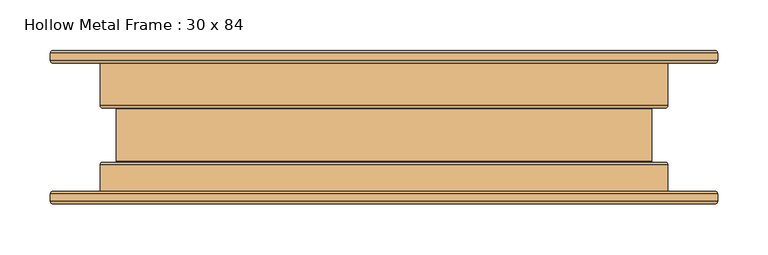
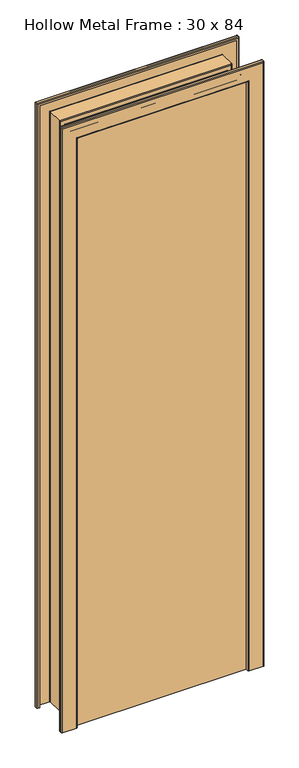
"""IFC4 building model written with IfcOpenShell, lengths in millimetres: door geometry, Hollow Metal Frame : 30 x 84."""

from ifc_helpers import new_model, si_unit, frame, origin, origin_with_axes, place, context, project, spatial, polyline, circle_curve, ellipse_curve, outline, extrude, source, transform, mapped, element, save
from ifc_brep_helpers import plane_surface, cylinder_surface, revolved_surface, advanced_brep


def hollow_metal_frame_30_x_84_32adf456(model_context):
    return source(origin(), model_context, "Body", "SolidModel", [
        advanced_brep(
        [(-327.62825, 63.5635, 0.0), (-330.2, 66.13525, 0.0), (-330.2, 73.66, 0.0), (-327.62825, 76.23175, 0.0), (-281.97175, 76.23175, 0.0), (-279.4, 73.66, 0.0), (-279.4, 21.68525, 0.0), (-278.384, 20.66925, 0.0), (-266.09675, 20.66925, 0.0), (-263.525, 18.0975, 0.0), (-263.525, -33.6931, 0.0), (-266.09675, -36.26485, 0.0), (-278.384, -36.26485, 0.0), (-279.4, -37.28085, 0.0), (-279.4, -73.5965, 0.0), (-281.97175, -76.16825, 0.0), (-327.62825, -76.16825, 0.0), (-330.2, -73.5965, 0.0), (-330.2, -66.07175, 0.0), (-327.62825, -63.5, 0.0), (-322.2625, -63.5, 0.0), (-322.2625, -65.05575, 0.0), (-327.62825, -65.05575, 0.0), (-328.64425, -66.07175, 0.0), (-328.64425, -73.5965, 0.0), (-327.62825, -74.6125, 0.0), (-281.97175, -74.6125, 0.0), (-280.95575, -73.5965, 0.0), (-280.95575, -37.28085, 0.0), (-278.384, -34.7091, 0.0), (-266.09675, -34.7091, 0.0), (-265.08075, -33.6931, 0.0), (-265.08075, 18.0975, 0.0), (-266.09675, 19.1135, 0.0), (-278.384, 19.1135, 0.0), (-280.95575, 21.68525, 0.0), (-280.95575, 73.66, 0.0), (-281.97175, 74.676, 0.0), (-327.62825, 74.676, 0.0), (-328.64425, 73.66, 0.0), (-328.64425, 66.13525, 0.0), (-327.62825, 65.11925, 0.0), (-322.2625, 65.11925, 0.0), (-322.2625, 63.5635, 0.0), (-327.62825, 63.5635, 2080.2282501), (-330.2, 66.13525, 2082.8000001), (-330.2, 73.66, 2082.8000001), (-327.62825, 76.23175, 2080.2282501), (327.62825, 76.23175, 2080.2282501), (327.62825, 76.23175, 0.0), (281.97175, 76.23175, 0.0), (281.97175, 76.23175, 2034.5717501), (-281.97175, 76.23175, 2034.5717501), (-279.4, 73.66, 2032.0000001), (-279.4, 21.68525, 2032.0000001), (-278.384, 20.66925, 2030.9840001), (278.384, 20.66925, 2030.9840001), (278.384, 20.66925, 0.0), (266.09675, 20.66925, 0.0), (266.09675, 20.66925, 2018.6967501), (-266.09675, 20.66925, 2018.6967501), (-263.525, 18.0975, 2016.1250001), (-263.525, -33.6931, 2016.1250001), (-266.09675, -36.26485, 2018.6967501), (266.09675, -36.26485, 2018.6967501), (266.09675, -36.26485, 0.0), (278.384, -36.26485, 0.0), (278.384, -36.26485, 2030.9840001), (-278.384, -36.26485, 2030.9840001), (-279.4, -37.28085, 2032.0000001), (-279.4, -73.5965, 2032.0000001), (-281.97175, -76.16825, 2034.5717501), (281.97175, -76.16825, 2034.5717501), (281.97175, -76.16825, 0.0), (327.62825, -76.16825, 0.0), (327.62825, -76.16825, 2080.2282501), (-327.62825, -76.16825, 2080.2282501), (-330.2, -73.5965, 2082.8000001), (-330.2, -66.07175, 2082.8000001), (-327.62825, -63.5, 2080.2282501), (327.62825, -63.5, 2080.2282501), (327.62825, -63.5, 0.0), (322.2625, -63.5, 0.0), (322.2625, -63.5, 2074.8625001), (-322.2625, -63.5, 2074.8625001), (-322.2625, -65.05575, 2074.8625001), (322.2625, -65.05575, 2074.8625001), (322.2625, -65.05575, 0.0), (327.62825, -65.05575, 0.0), (327.62825, -65.05575, 2080.2282501), (-327.62825, -65.05575, 2080.2282501), (-328.64425, -66.07175, 2081.2442501), (-328.64425, -73.5965, 2081.2442501), (-327.62825, -74.6125, 2080.2282501), (327.62825, -74.6125, 2080.2282501), (327.62825, -74.6125, 0.0), (281.97175, -74.6125, 0.0), (281.97175, -74.6125, 2034.5717501), (-281.97175, -74.6125, 2034.5717501), (-280.95575, -73.5965, 2033.5557501), (-280.95575, -37.28085, 2033.5557501), (-278.384, -34.7091, 2030.9840001), (278.384, -34.7091, 2030.9840001), (278.384, -34.7091, 0.0), (266.09675, -34.7091, 0.0), (266.09675, -34.7091, 2018.6967501), (-266.09675, -34.7091, 2018.6967501), (-265.08075, -33.6931, 2017.6807501), (-265.08075, 18.0975, 2017.6807501), (-266.09675, 19.1135, 2018.6967501), (266.09675, 19.1135, 2018.6967501), (266.09675, 19.1135, 0.0), (278.384, 19.1135, 0.0), (278.384, 19.1135, 2030.9840001), (-278.384, 19.1135, 2030.9840001), (-280.95575, 21.68525, 2033.5557501), (-280.95575, 73.66, 2033.5557501), (-281.97175, 74.676, 2034.5717501), (281.97175, 74.676, 2034.5717501), (281.97175, 74.676, 0.0), (327.62825, 74.676, 0.0), (327.62825, 74.676, 2080.2282501), (-327.62825, 74.676, 2080.2282501), (-328.64425, 73.66, 2081.2442501), (-328.64425, 66.13525, 2081.2442501), (-327.62825, 65.11925, 2080.2282501), (327.62825, 65.11925, 2080.2282501), (327.62825, 65.11925, 0.0), (322.2625, 65.11925, 0.0), (322.2625, 65.11925, 2074.8625001), (-322.2625, 65.11925, 2074.8625001), (-322.2625, 63.5635, 2074.8625001), (322.2625, 63.5635, 2074.8625001), (322.2625, 63.5635, 0.0), (327.62825, 63.5635, 0.0), (327.62825, 63.5635, 2080.2282501), (330.2, 66.13525, 2082.8000001), (330.2, 73.66, 2082.8000001), (279.4, 73.66, 2032.0000001), (279.4, 21.68525, 2032.0000001), (263.525, 18.0975, 2016.1250001), (263.525, -33.6931, 2016.1250001), (279.4, -37.28085, 2032.0000001), (279.4, -73.5965, 2032.0000001), (330.2, -73.5965, 2082.8000001), (330.2, -66.07175, 2082.8000001), (328.64425, -66.07175, 2081.2442501), (328.64425, -73.5965, 2081.2442501), (280.95575, -73.5965, 2033.5557501), (280.95575, -37.28085, 2033.5557501), (265.08075, -33.6931, 2017.6807501), (265.08075, 18.0975, 2017.6807501), (280.95575, 21.68525, 2033.5557501), (280.95575, 73.66, 2033.5557501), (328.64425, 73.66, 2081.2442501), (328.64425, 66.13525, 2081.2442501), (328.64425, 66.13525, 0.0), (328.64425, 73.66, 0.0), (280.95575, 73.66, 0.0), (280.95575, 21.68525, 0.0), (265.08075, 18.0975, 0.0), (265.08075, -33.6931, 0.0), (280.95575, -37.28085, 0.0), (280.95575, -73.5965, 0.0), (328.64425, -73.5965, 0.0), (328.64425, -66.07175, 0.0), (330.2, -66.07175, 0.0), (330.2, -73.5965, 0.0), (279.4, -73.5965, 0.0), (279.4, -37.28085, 0.0), (263.525, -33.6931, 0.0), (263.525, 18.0975, 0.0), (279.4, 21.68525, 0.0), (279.4, 73.66, 0.0), (330.2, 73.66, 0.0), (330.2, 66.13525, 0.0)],
        [
            (0, 1, circle_curve(frame((-327.62825, 66.13525, 0.0), z_axis=(0.0, 0.0, -1.0), x_axis=(0.0, -1.0, 0.0)), 2.57175)),
            (1, 2),
            (2, 3, circle_curve(frame((-327.62825, 73.66, 0.0), z_axis=(0.0, 0.0, -1.0), x_axis=(0.0, -1.0, 0.0)), 2.57175)),
            (3, 4),
            (4, 5, circle_curve(frame((-281.97175, 73.66, 0.0), z_axis=(0.0, 0.0, -1.0), x_axis=(0.0, -1.0, 0.0)), 2.57175)),
            (5, 6),
            (6, 7, circle_curve(frame((-278.384, 21.68525, 0.0), z_axis=(0.0, 0.0, 1.0), x_axis=(0.0, -1.0, 0.0)), 1.016)),
            (7, 8),
            (8, 9, circle_curve(frame((-266.09675, 18.0975, 0.0), z_axis=(0.0, 0.0, -1.0), x_axis=(0.0, -1.0, 0.0)), 2.57175)),
            (9, 10),
            (10, 11, circle_curve(frame((-266.09675, -33.6931, 0.0), z_axis=(0.0, 0.0, -1.0), x_axis=(0.0, -1.0, 0.0)), 2.57175)),
            (11, 12),
            (12, 13, circle_curve(frame((-278.384, -37.28085, 0.0), z_axis=(0.0, 0.0, 1.0), x_axis=(0.0, -1.0, 0.0)), 1.016)),
            (13, 14),
            (14, 15, circle_curve(frame((-281.97175, -73.5965, 0.0), z_axis=(0.0, 0.0, -1.0), x_axis=(0.0, -1.0, 0.0)), 2.57175)),
            (15, 16),
            (16, 17, circle_curve(frame((-327.62825, -73.5965, 0.0), z_axis=(0.0, 0.0, -1.0), x_axis=(0.0, -1.0, 0.0)), 2.57175)),
            (17, 18),
            (18, 19, circle_curve(frame((-327.62825, -66.07175, 0.0), z_axis=(0.0, 0.0, -1.0), x_axis=(0.0, -1.0, 0.0)), 2.57175)),
            (19, 20),
            (20, 21),
            (21, 22),
            (22, 23, circle_curve(frame((-327.62825, -66.07175, 0.0), z_axis=(0.0, 0.0, 1.0), x_axis=(0.0, -1.0, 0.0)), 1.016)),
            (23, 24),
            (24, 25, circle_curve(frame((-327.62825, -73.5965, 0.0), z_axis=(0.0, 0.0, 1.0), x_axis=(0.0, -1.0, 0.0)), 1.016)),
            (25, 26),
            (26, 27, circle_curve(frame((-281.97175, -73.5965, 0.0), z_axis=(0.0, 0.0, 1.0), x_axis=(0.0, -1.0, 0.0)), 1.016)),
            (27, 28),
            (28, 29, circle_curve(frame((-278.384, -37.28085, 0.0), z_axis=(0.0, 0.0, -1.0), x_axis=(0.0, -1.0, 0.0)), 2.57175)),
            (29, 30),
            (30, 31, circle_curve(frame((-266.09675, -33.6931, 0.0), z_axis=(0.0, 0.0, 1.0), x_axis=(0.0, -1.0, 0.0)), 1.016)),
            (31, 32),
            (32, 33, circle_curve(frame((-266.09675, 18.0975, 0.0), z_axis=(0.0, 0.0, 1.0), x_axis=(0.0, -1.0, 0.0)), 1.016)),
            (33, 34),
            (34, 35, circle_curve(frame((-278.384, 21.68525, 0.0), z_axis=(0.0, 0.0, -1.0), x_axis=(0.0, -1.0, 0.0)), 2.57175)),
            (35, 36),
            (36, 37, circle_curve(frame((-281.97175, 73.66, 0.0), z_axis=(0.0, 0.0, 1.0), x_axis=(0.0, -1.0, 0.0)), 1.016)),
            (37, 38),
            (38, 39, circle_curve(frame((-327.62825, 73.66, 0.0), z_axis=(0.0, 0.0, 1.0), x_axis=(0.0, -1.0, 0.0)), 1.016)),
            (39, 40),
            (40, 41, circle_curve(frame((-327.62825, 66.13525, 0.0), z_axis=(0.0, 0.0, 1.0), x_axis=(0.0, -1.0, 0.0)), 1.016)),
            (41, 42),
            (42, 43),
            (43, 0),
            (0, 44),
            (44, 45, ellipse_curve(frame((-327.62825, 66.13525, 2080.2282501), z_axis=(-0.7071067811865475, 0.0, -0.7071067811865475), x_axis=(0.7071067811865474, 0.0, -0.7071067811865476)), 3.6370037, 2.57175)),
            (45, 1),
            (45, 46),
            (46, 2),
            (46, 47, ellipse_curve(frame((-327.62825, 73.66, 2080.2282501), z_axis=(-0.7071067811865475, 0.0, -0.7071067811865475), x_axis=(0.7071067811865474, 0.0, -0.7071067811865476)), 3.6370037, 2.57175)),
            (47, 3),
            (47, 48),
            (48, 49),
            (49, 50),
            (50, 51),
            (51, 52),
            (52, 4),
            (52, 53, ellipse_curve(frame((-281.97175, 73.66, 2034.5717501), z_axis=(-0.7071067811865475, 0.0, -0.7071067811865475), x_axis=(0.7071067811865474, 0.0, -0.7071067811865476)), 3.6370037, 2.57175)),
            (53, 5),
            (53, 54),
            (54, 6),
            (54, 55, ellipse_curve(frame((-278.384, 21.68525, 2030.9840001), z_axis=(0.7071067811865475, 0.0, 0.7071067811865475), x_axis=(-0.7071067811865474, 0.0, 0.7071067811865476)), 1.436841, 1.016)),
            (55, 7),
            (55, 56),
            (56, 57),
            (57, 58),
            (58, 59),
            (59, 60),
            (60, 8),
            (60, 61, ellipse_curve(frame((-266.09675, 18.0975, 2018.6967501), z_axis=(-0.7071067811865475, 0.0, -0.7071067811865475), x_axis=(0.7071067811865474, 0.0, -0.7071067811865476)), 3.6370037, 2.57175)),
            (61, 9),
            (61, 62),
            (62, 10),
            (62, 63, ellipse_curve(frame((-266.09675, -33.6931, 2018.6967501), z_axis=(-0.7071067811865475, 0.0, -0.7071067811865475), x_axis=(0.7071067811865474, 0.0, -0.7071067811865476)), 3.6370037, 2.57175)),
            (63, 11),
            (63, 64),
            (64, 65),
            (65, 66),
            (66, 67),
            (67, 68),
            (68, 12),
            (68, 69, ellipse_curve(frame((-278.384, -37.28085, 2030.9840001), z_axis=(0.7071067811865475, 0.0, 0.7071067811865475), x_axis=(-0.7071067811865474, 0.0, 0.7071067811865476)), 1.436841, 1.016)),
            (69, 13),
            (69, 70),
            (70, 14),
            (70, 71, ellipse_curve(frame((-281.97175, -73.5965, 2034.5717501), z_axis=(-0.7071067811865475, 0.0, -0.7071067811865475), x_axis=(0.7071067811865474, 0.0, -0.7071067811865476)), 3.6370037, 2.57175)),
            (71, 15),
            (71, 72),
            (72, 73),
            (73, 74),
            (74, 75),
            (75, 76),
            (76, 16),
            (76, 77, ellipse_curve(frame((-327.62825, -73.5965, 2080.2282501), z_axis=(-0.7071067811865475, 0.0, -0.7071067811865475), x_axis=(0.7071067811865474, 0.0, -0.7071067811865476)), 3.6370037, 2.57175)),
            (77, 17),
            (77, 78),
            (78, 18),
            (78, 79, ellipse_curve(frame((-327.62825, -66.07175, 2080.2282501), z_axis=(-0.7071067811865475, 0.0, -0.7071067811865475), x_axis=(0.7071067811865474, 0.0, -0.7071067811865476)), 3.6370037, 2.57175)),
            (79, 19),
            (79, 80),
            (80, 81),
            (81, 82),
            (82, 83),
            (83, 84),
            (84, 20),
            (84, 85),
            (85, 21),
            (85, 86),
            (86, 87),
            (87, 88),
            (88, 89),
            (89, 90),
            (90, 22),
            (90, 91, ellipse_curve(frame((-327.62825, -66.07175, 2080.2282501), z_axis=(0.7071067811865475, 0.0, 0.7071067811865475), x_axis=(-0.7071067811865474, 0.0, 0.7071067811865476)), 1.436841, 1.016)),
            (91, 23),
            (91, 92),
            (92, 24),
            (92, 93, ellipse_curve(frame((-327.62825, -73.5965, 2080.2282501), z_axis=(0.7071067811865475, 0.0, 0.7071067811865475), x_axis=(-0.7071067811865474, 0.0, 0.7071067811865476)), 1.436841, 1.016)),
            (93, 25),
            (93, 94),
            (94, 95),
            (95, 96),
            (96, 97),
            (97, 98),
            (98, 26),
            (98, 99, ellipse_curve(frame((-281.97175, -73.5965, 2034.5717501), z_axis=(0.7071067811865475, 0.0, 0.7071067811865475), x_axis=(-0.7071067811865474, 0.0, 0.7071067811865476)), 1.436841, 1.016)),
            (99, 27),
            (99, 100),
            (100, 28),
            (100, 101, ellipse_curve(frame((-278.384, -37.28085, 2030.9840001), z_axis=(-0.7071067811865475, 0.0, -0.7071067811865475), x_axis=(0.7071067811865474, 0.0, -0.7071067811865476)), 3.6370037, 2.57175)),
            (101, 29),
            (101, 102),
            (102, 103),
            (103, 104),
            (104, 105),
            (105, 106),
            (106, 30),
            (106, 107, ellipse_curve(frame((-266.09675, -33.6931, 2018.6967501), z_axis=(0.7071067811865475, 0.0, 0.7071067811865475), x_axis=(-0.7071067811865474, 0.0, 0.7071067811865476)), 1.436841, 1.016)),
            (107, 31),
            (107, 108),
            (108, 32),
            (108, 109, ellipse_curve(frame((-266.09675, 18.0975, 2018.6967501), z_axis=(0.7071067811865475, 0.0, 0.7071067811865475), x_axis=(-0.7071067811865474, 0.0, 0.7071067811865476)), 1.436841, 1.016)),
            (109, 33),
            (109, 110),
            (110, 111),
            (111, 112),
            (112, 113),
            (113, 114),
            (114, 34),
            (114, 115, ellipse_curve(frame((-278.384, 21.68525, 2030.9840001), z_axis=(-0.7071067811865475, 0.0, -0.7071067811865475), x_axis=(0.7071067811865474, 0.0, -0.7071067811865476)), 3.6370037, 2.57175)),
            (115, 35),
            (115, 116),
            (116, 36),
            (116, 117, ellipse_curve(frame((-281.97175, 73.66, 2034.5717501), z_axis=(0.7071067811865475, 0.0, 0.7071067811865475), x_axis=(-0.7071067811865474, 0.0, 0.7071067811865476)), 1.436841, 1.016)),
            (117, 37),
            (117, 118),
            (118, 119),
            (119, 120),
            (120, 121),
            (121, 122),
            (122, 38),
            (122, 123, ellipse_curve(frame((-327.62825, 73.66, 2080.2282501), z_axis=(0.7071067811865475, 0.0, 0.7071067811865475), x_axis=(-0.7071067811865474, 0.0, 0.7071067811865476)), 1.436841, 1.016)),
            (123, 39),
            (123, 124),
            (124, 40),
            (124, 125, ellipse_curve(frame((-327.62825, 66.13525, 2080.2282501), z_axis=(0.7071067811865475, 0.0, 0.7071067811865475), x_axis=(-0.7071067811865474, 0.0, 0.7071067811865476)), 1.436841, 1.016)),
            (125, 41),
            (125, 126),
            (126, 127),
            (127, 128),
            (128, 129),
            (129, 130),
            (130, 42),
            (130, 131),
            (131, 43),
            (131, 132),
            (132, 133),
            (133, 134),
            (134, 135),
            (135, 44),
            (135, 136, ellipse_curve(frame((327.62825, 66.13525, 2080.2282501), z_axis=(-0.7071067811865475, 0.0, 0.7071067811865475), x_axis=(-0.7071067811865476, 0.0, -0.7071067811865474)), 3.6370037, 2.57175)),
            (136, 45),
            (136, 137),
            (137, 46),
            (137, 48, ellipse_curve(frame((327.62825, 73.66, 2080.2282501), z_axis=(-0.7071067811865475, 0.0, 0.7071067811865475), x_axis=(-0.7071067811865476, 0.0, -0.7071067811865474)), 3.6370037, 2.57175)),
            (51, 138, ellipse_curve(frame((281.97175, 73.66, 2034.5717501), z_axis=(-0.7071067811865475, 0.0, 0.7071067811865475), x_axis=(-0.7071067811865476, 0.0, -0.7071067811865474)), 3.6370037, 2.57175)),
            (138, 53),
            (138, 139),
            (139, 54),
            (139, 56, ellipse_curve(frame((278.384, 21.68525, 2030.9840001), z_axis=(0.7071067811865475, 0.0, -0.7071067811865475), x_axis=(0.7071067811865476, 0.0, 0.7071067811865474)), 1.436841, 1.016)),
            (59, 140, ellipse_curve(frame((266.09675, 18.0975, 2018.6967501), z_axis=(-0.7071067811865475, 0.0, 0.7071067811865475), x_axis=(-0.7071067811865476, 0.0, -0.7071067811865474)), 3.6370037, 2.57175)),
            (140, 61),
            (140, 141),
            (141, 62),
            (141, 64, ellipse_curve(frame((266.09675, -33.6931, 2018.6967501), z_axis=(-0.7071067811865475, 0.0, 0.7071067811865475), x_axis=(-0.7071067811865476, 0.0, -0.7071067811865474)), 3.6370037, 2.57175)),
            (67, 142, ellipse_curve(frame((278.384, -37.28085, 2030.9840001), z_axis=(0.7071067811865475, 0.0, -0.7071067811865475), x_axis=(0.7071067811865476, 0.0, 0.7071067811865474)), 1.436841, 1.016)),
            (142, 69),
            (142, 143),
            (143, 70),
            (143, 72, ellipse_curve(frame((281.97175, -73.5965, 2034.5717501), z_axis=(-0.7071067811865475, 0.0, 0.7071067811865475), x_axis=(-0.7071067811865476, 0.0, -0.7071067811865474)), 3.6370037, 2.57175)),
            (75, 144, ellipse_curve(frame((327.62825, -73.5965, 2080.2282501), z_axis=(-0.7071067811865475, 0.0, 0.7071067811865475), x_axis=(-0.7071067811865476, 0.0, -0.7071067811865474)), 3.6370037, 2.57175)),
            (144, 77),
            (144, 145),
            (145, 78),
            (145, 80, ellipse_curve(frame((327.62825, -66.07175, 2080.2282501), z_axis=(-0.7071067811865475, 0.0, 0.7071067811865475), x_axis=(-0.7071067811865476, 0.0, -0.7071067811865474)), 3.6370037, 2.57175)),
            (83, 86),
            (89, 146, ellipse_curve(frame((327.62825, -66.07175, 2080.2282501), z_axis=(0.7071067811865475, 0.0, -0.7071067811865475), x_axis=(0.7071067811865476, 0.0, 0.7071067811865474)), 1.436841, 1.016)),
            (146, 91),
            (146, 147),
            (147, 92),
            (147, 94, ellipse_curve(frame((327.62825, -73.5965, 2080.2282501), z_axis=(0.7071067811865475, 0.0, -0.7071067811865475), x_axis=(0.7071067811865476, 0.0, 0.7071067811865474)), 1.436841, 1.016)),
            (97, 148, ellipse_curve(frame((281.97175, -73.5965, 2034.5717501), z_axis=(0.7071067811865475, 0.0, -0.7071067811865475), x_axis=(0.7071067811865476, 0.0, 0.7071067811865474)), 1.436841, 1.016)),
            (148, 99),
            (148, 149),
            (149, 100),
            (149, 102, ellipse_curve(frame((278.384, -37.28085, 2030.9840001), z_axis=(-0.7071067811865475, 0.0, 0.7071067811865475), x_axis=(-0.7071067811865476, 0.0, -0.7071067811865474)), 3.6370037, 2.57175)),
            (105, 150, ellipse_curve(frame((266.09675, -33.6931, 2018.6967501), z_axis=(0.7071067811865475, 0.0, -0.7071067811865475), x_axis=(0.7071067811865476, 0.0, 0.7071067811865474)), 1.436841, 1.016)),
            (150, 107),
            (150, 151),
            (151, 108),
            (151, 110, ellipse_curve(frame((266.09675, 18.0975, 2018.6967501), z_axis=(0.7071067811865475, 0.0, -0.7071067811865475), x_axis=(0.7071067811865476, 0.0, 0.7071067811865474)), 1.436841, 1.016)),
            (113, 152, ellipse_curve(frame((278.384, 21.68525, 2030.9840001), z_axis=(-0.7071067811865475, 0.0, 0.7071067811865475), x_axis=(-0.7071067811865476, 0.0, -0.7071067811865474)), 3.6370037, 2.57175)),
            (152, 115),
            (152, 153),
            (153, 116),
            (153, 118, ellipse_curve(frame((281.97175, 73.66, 2034.5717501), z_axis=(0.7071067811865475, 0.0, -0.7071067811865475), x_axis=(0.7071067811865476, 0.0, 0.7071067811865474)), 1.436841, 1.016)),
            (121, 154, ellipse_curve(frame((327.62825, 73.66, 2080.2282501), z_axis=(0.7071067811865475, 0.0, -0.7071067811865475), x_axis=(0.7071067811865476, 0.0, 0.7071067811865474)), 1.436841, 1.016)),
            (154, 123),
            (154, 155),
            (155, 124),
            (155, 126, ellipse_curve(frame((327.62825, 66.13525, 2080.2282501), z_axis=(0.7071067811865475, 0.0, -0.7071067811865475), x_axis=(0.7071067811865476, 0.0, 0.7071067811865474)), 1.436841, 1.016)),
            (129, 132),
            (133, 128),
            (127, 156, circle_curve(frame((327.62825, 66.13525, 0.0), z_axis=(0.0, 0.0, 1.0), x_axis=(0.0, -1.0, 0.0)), 1.016)),
            (156, 157),
            (157, 120, circle_curve(frame((327.62825, 73.66, 0.0), z_axis=(0.0, 0.0, 1.0), x_axis=(0.0, -1.0, 0.0)), 1.016)),
            (119, 158, circle_curve(frame((281.97175, 73.66, 0.0), z_axis=(0.0, 0.0, 1.0), x_axis=(0.0, -1.0, 0.0)), 1.016)),
            (158, 159),
            (159, 112, circle_curve(frame((278.384, 21.68525, 0.0), z_axis=(0.0, 0.0, -1.0), x_axis=(0.0, -1.0, 0.0)), 2.57175)),
            (111, 160, circle_curve(frame((266.09675, 18.0975, 0.0), z_axis=(0.0, 0.0, 1.0), x_axis=(0.0, -1.0, 0.0)), 1.016)),
            (160, 161),
            (161, 104, circle_curve(frame((266.09675, -33.6931, 0.0), z_axis=(0.0, 0.0, 1.0), x_axis=(0.0, -1.0, 0.0)), 1.016)),
            (103, 162, circle_curve(frame((278.384, -37.28085, 0.0), z_axis=(0.0, 0.0, -1.0), x_axis=(0.0, -1.0, 0.0)), 2.57175)),
            (162, 163),
            (163, 96, circle_curve(frame((281.97175, -73.5965, 0.0), z_axis=(0.0, 0.0, 1.0), x_axis=(0.0, -1.0, 0.0)), 1.016)),
            (95, 164, circle_curve(frame((327.62825, -73.5965, 0.0), z_axis=(0.0, 0.0, 1.0), x_axis=(0.0, -1.0, 0.0)), 1.016)),
            (164, 165),
            (165, 88, circle_curve(frame((327.62825, -66.07175, 0.0), z_axis=(0.0, 0.0, 1.0), x_axis=(0.0, -1.0, 0.0)), 1.016)),
            (87, 82),
            (81, 166, circle_curve(frame((327.62825, -66.07175, 0.0), z_axis=(0.0, 0.0, -1.0), x_axis=(0.0, -1.0, 0.0)), 2.57175)),
            (166, 167),
            (167, 74, circle_curve(frame((327.62825, -73.5965, 0.0), z_axis=(0.0, 0.0, -1.0), x_axis=(0.0, -1.0, 0.0)), 2.57175)),
            (73, 168, circle_curve(frame((281.97175, -73.5965, 0.0), z_axis=(0.0, 0.0, -1.0), x_axis=(0.0, -1.0, 0.0)), 2.57175)),
            (168, 169),
            (169, 66, circle_curve(frame((278.384, -37.28085, 0.0), z_axis=(0.0, 0.0, 1.0), x_axis=(0.0, -1.0, 0.0)), 1.016)),
            (65, 170, circle_curve(frame((266.09675, -33.6931, 0.0), z_axis=(0.0, 0.0, -1.0), x_axis=(0.0, -1.0, 0.0)), 2.57175)),
            (170, 171),
            (171, 58, circle_curve(frame((266.09675, 18.0975, 0.0), z_axis=(0.0, 0.0, -1.0), x_axis=(0.0, -1.0, 0.0)), 2.57175)),
            (57, 172, circle_curve(frame((278.384, 21.68525, 0.0), z_axis=(0.0, 0.0, 1.0), x_axis=(0.0, -1.0, 0.0)), 1.016)),
            (172, 173),
            (173, 50, circle_curve(frame((281.97175, 73.66, 0.0), z_axis=(0.0, 0.0, -1.0), x_axis=(0.0, -1.0, 0.0)), 2.57175)),
            (49, 174, circle_curve(frame((327.62825, 73.66, 0.0), z_axis=(0.0, 0.0, -1.0), x_axis=(0.0, -1.0, 0.0)), 2.57175)),
            (174, 175),
            (175, 134, circle_curve(frame((327.62825, 66.13525, 0.0), z_axis=(0.0, 0.0, -1.0), x_axis=(0.0, -1.0, 0.0)), 2.57175)),
            (175, 136),
            (174, 137),
            (173, 138),
            (172, 139),
            (171, 140),
            (170, 141),
            (169, 142),
            (168, 143),
            (167, 144),
            (166, 145),
            (165, 146),
            (164, 147),
            (163, 148),
            (162, 149),
            (161, 150),
            (160, 151),
            (159, 152),
            (158, 153),
            (157, 154),
            (156, 155),
        ],
        [
            plane_surface(frame((-290.5125, -63.5, 0.0), z_axis=(0.0, 0.0, -1.0), x_axis=(1.0, 0.0, 0.0))),
            cylinder_surface(frame((-327.62825, 66.13525, 0.0), z_axis=(0.0, 0.0, -1.0), x_axis=(0.0, -1.0, 0.0)), 2.57175),
            plane_surface(frame((-330.2, 66.13525, 0.0), z_axis=(-1.0, 0.0, 0.0), x_axis=(0.0, 0.0, 1.0))),
            cylinder_surface(frame((-327.62825, 73.66, 0.0), z_axis=(0.0, 0.0, -1.0), x_axis=(0.0, -1.0, 0.0)), 2.57175),
            plane_surface(frame((-327.62825, 76.23175, 0.0), z_axis=(0.0, 1.0, 0.0), x_axis=(0.0, 0.0, 1.0))),
            cylinder_surface(frame((-281.97175, 73.66, 0.0), z_axis=(0.0, 0.0, -1.0), x_axis=(0.0, -1.0, 0.0)), 2.57175),
            plane_surface(frame((-279.4, 73.66, 0.0), z_axis=(1.0, 0.0, 0.0), x_axis=(0.0, 0.0, 1.0))),
            revolved_surface(polyline([(-278.384, 20.669249999999998, 2032.0000001145868), (-278.384, 20.669249999999998, 0.0)]), (-278.384, 21.68525, 0.0), (0.0, 0.0, 1.0)),
            plane_surface(frame((-278.384, 20.66925, 0.0), z_axis=(0.0, 1.0, 0.0), x_axis=(0.0, 0.0, 1.0))),
            cylinder_surface(frame((-266.09675, 18.0975, 0.0), z_axis=(0.0, 0.0, -1.0), x_axis=(0.0, -1.0, 0.0)), 2.57175),
            plane_surface(frame((-263.525, 18.0975, 0.0), z_axis=(1.0, 0.0, 0.0), x_axis=(0.0, 0.0, 1.0))),
            cylinder_surface(frame((-266.09675, -33.6931, 0.0), z_axis=(0.0, 0.0, -1.0), x_axis=(0.0, -1.0, 0.0)), 2.57175),
            plane_surface(frame((-266.09675, -36.26485, 0.0), z_axis=(0.0, -1.0, 0.0), x_axis=(0.0, 0.0, 1.0))),
            revolved_surface(polyline([(-278.384, -38.29685, 2032.0000001145868), (-278.384, -38.29685, 0.0)]), (-278.384, -37.28085, 0.0), (0.0, 0.0, 1.0)),
            plane_surface(frame((-279.4, -37.28085, 0.0), z_axis=(1.0, 0.0, 0.0), x_axis=(0.0, 0.0, 1.0))),
            cylinder_surface(frame((-281.97175, -73.5965, 0.0), z_axis=(0.0, 0.0, -1.0), x_axis=(0.0, -1.0, 0.0)), 2.57175),
            plane_surface(frame((-281.97175, -76.16825, 0.0), z_axis=(0.0, -1.0, 0.0), x_axis=(0.0, 0.0, 1.0))),
            cylinder_surface(frame((-327.62825, -73.5965, 0.0), z_axis=(0.0, 0.0, -1.0), x_axis=(0.0, -1.0, 0.0)), 2.57175),
            plane_surface(frame((-330.2, -73.5965, 0.0), z_axis=(-1.0, 0.0, 0.0), x_axis=(0.0, 0.0, 1.0))),
            cylinder_surface(frame((-327.62825, -66.07175, 0.0), z_axis=(0.0, 0.0, -1.0), x_axis=(0.0, -1.0, 0.0)), 2.57175),
            plane_surface(frame((-327.62825, -63.5, 0.0), z_axis=(0.0, 1.0, 0.0), x_axis=(0.0, 0.0, 1.0))),
            plane_surface(frame((-322.2625, -63.5, 0.0), z_axis=(1.0, 0.0, 0.0), x_axis=(0.0, 0.0, 1.0))),
            plane_surface(frame((-322.2625, -65.05575, 0.0), z_axis=(0.0, -1.0, 0.0), x_axis=(0.0, 0.0, 1.0))),
            revolved_surface(polyline([(-327.62825, -67.08775, 2081.244250114587), (-327.62825, -67.08775, 0.0)]), (-327.62825, -66.07175, 0.0), (0.0, 0.0, 1.0)),
            plane_surface(frame((-328.64425, -66.07175, 0.0), z_axis=(1.0, 0.0, 0.0), x_axis=(0.0, 0.0, 1.0))),
            revolved_surface(polyline([(-327.62825, -74.61250000000001, 2081.244250114587), (-327.62825, -74.61250000000001, 0.0)]), (-327.62825, -73.5965, 0.0), (0.0, 0.0, 1.0)),
            plane_surface(frame((-327.62825, -74.6125, 0.0), z_axis=(0.0, 1.0, 0.0), x_axis=(0.0, 0.0, 1.0))),
            revolved_surface(polyline([(-281.97175, -74.61250000000001, 2035.5877501145867), (-281.97175, -74.61250000000001, 0.0)]), (-281.97175, -73.5965, 0.0), (0.0, 0.0, 1.0)),
            plane_surface(frame((-280.95575, -73.5965, 0.0), z_axis=(-1.0, 0.0, 0.0), x_axis=(0.0, 0.0, 1.0))),
            cylinder_surface(frame((-278.384, -37.28085, 0.0), z_axis=(0.0, 0.0, -1.0), x_axis=(0.0, -1.0, 0.0)), 2.57175),
            plane_surface(frame((-278.384, -34.7091, 0.0), z_axis=(0.0, 1.0, 0.0), x_axis=(0.0, 0.0, 1.0))),
            revolved_surface(polyline([(-266.09675, -34.7091, 2019.7127501145867), (-266.09675, -34.7091, 0.0)]), (-266.09675, -33.6931, 0.0), (0.0, 0.0, 1.0)),
            plane_surface(frame((-265.08075, -33.6931, 0.0), z_axis=(-1.0, 0.0, 0.0), x_axis=(0.0, 0.0, 1.0))),
            revolved_surface(polyline([(-266.09675, 17.0815, 2019.7127501145867), (-266.09675, 17.0815, 0.0)]), (-266.09675, 18.0975, 0.0), (0.0, 0.0, 1.0)),
            plane_surface(frame((-266.09675, 19.1135, 0.0), z_axis=(0.0, -1.0, 0.0), x_axis=(0.0, 0.0, 1.0))),
            cylinder_surface(frame((-278.384, 21.68525, 0.0), z_axis=(0.0, 0.0, -1.0), x_axis=(0.0, -1.0, 0.0)), 2.57175),
            plane_surface(frame((-280.95575, 21.68525, 0.0), z_axis=(-1.0, 0.0, 0.0), x_axis=(0.0, 0.0, 1.0))),
            revolved_surface(polyline([(-281.97175, 72.64399999999999, 2035.5877501145867), (-281.97175, 72.64399999999999, 0.0)]), (-281.97175, 73.66, 0.0), (0.0, 0.0, 1.0)),
            plane_surface(frame((-281.97175, 74.676, 0.0), z_axis=(0.0, -1.0, 0.0), x_axis=(0.0, 0.0, 1.0))),
            revolved_surface(polyline([(-327.62825, 72.64399999999999, 2081.244250114587), (-327.62825, 72.64399999999999, 0.0)]), (-327.62825, 73.66, 0.0), (0.0, 0.0, 1.0)),
            plane_surface(frame((-328.64425, 73.66, 0.0), z_axis=(1.0, 0.0, 0.0), x_axis=(0.0, 0.0, 1.0))),
            revolved_surface(polyline([(-327.62825, 65.11925, 2081.244250114587), (-327.62825, 65.11925, 0.0)]), (-327.62825, 66.13525, 0.0), (0.0, 0.0, 1.0)),
            plane_surface(frame((-327.62825, 65.11925, 0.0), z_axis=(0.0, 1.0, 0.0), x_axis=(0.0, 0.0, 1.0))),
            plane_surface(frame((-322.2625, 65.11925, 0.0), z_axis=(1.0, 0.0, 0.0), x_axis=(0.0, 0.0, 1.0))),
            plane_surface(frame((-322.2625, 63.5635, 0.0), z_axis=(0.0, -1.0, 0.0), x_axis=(0.0, 0.0, 1.0))),
            cylinder_surface(frame((-290.5125, 66.13525, 2080.2282501), z_axis=(-1.0, 0.0, 0.0), x_axis=(0.0, -1.0, 0.0)), 2.57175),
            plane_surface(frame((-330.2, 66.13525, 2082.8000001), z_axis=(0.0, 0.0, 1.0), x_axis=(1.0, 0.0, 0.0))),
            cylinder_surface(frame((-290.5125, 73.66, 2080.2282501), z_axis=(-1.0, 0.0, 0.0), x_axis=(0.0, -1.0, 0.0)), 2.57175),
            cylinder_surface(frame((-290.5125, 73.66, 2034.5717501), z_axis=(-1.0, 0.0, 0.0), x_axis=(0.0, -1.0, 0.0)), 2.57175),
            plane_surface(frame((-279.4, 73.66, 2032.0000001), z_axis=(0.0, 0.0, -1.0), x_axis=(1.0, 0.0, 0.0))),
            revolved_surface(polyline([(279.40000001458696, 20.669249999999998, 2030.9840001), (-279.40000001458685, 20.669249999999998, 2030.9840001)]), (-290.5125, 21.68525, 2030.9840001), (1.0, 0.0, 0.0)),
            cylinder_surface(frame((-290.5125, 18.0975, 2018.6967501), z_axis=(-1.0, 0.0, 0.0), x_axis=(0.0, -1.0, 0.0)), 2.57175),
            plane_surface(frame((-263.525, 18.0975, 2016.1250001), z_axis=(0.0, 0.0, -1.0), x_axis=(1.0, 0.0, 0.0))),
            cylinder_surface(frame((-290.5125, -33.6931, 2018.6967501), z_axis=(-1.0, 0.0, 0.0), x_axis=(0.0, -1.0, 0.0)), 2.57175),
            revolved_surface(polyline([(279.40000001458696, -38.29685, 2030.9840001), (-279.40000001458685, -38.29685, 2030.9840001)]), (-290.5125, -37.28085, 2030.9840001), (1.0, 0.0, 0.0)),
            plane_surface(frame((-279.4, -37.28085, 2032.0000001), z_axis=(0.0, 0.0, -1.0), x_axis=(1.0, 0.0, 0.0))),
            cylinder_surface(frame((-290.5125, -73.5965, 2034.5717501), z_axis=(-1.0, 0.0, 0.0), x_axis=(0.0, -1.0, 0.0)), 2.57175),
            cylinder_surface(frame((-290.5125, -73.5965, 2080.2282501), z_axis=(-1.0, 0.0, 0.0), x_axis=(0.0, -1.0, 0.0)), 2.57175),
            plane_surface(frame((-330.2, -73.5965, 2082.8000001), z_axis=(0.0, 0.0, 1.0), x_axis=(1.0, 0.0, 0.0))),
            cylinder_surface(frame((-290.5125, -66.07175, 2080.2282501), z_axis=(-1.0, 0.0, 0.0), x_axis=(0.0, -1.0, 0.0)), 2.57175),
            plane_surface(frame((-322.2625, -63.5, 2074.8625001), z_axis=(0.0, 0.0, -1.0), x_axis=(1.0, 0.0, 0.0))),
            revolved_surface(polyline([(328.64425001458693, -67.08775, 2080.2282501), (-328.6442500145868, -67.08775, 2080.2282501)]), (-290.5125, -66.07175, 2080.2282501), (1.0, 0.0, 0.0)),
            plane_surface(frame((-328.64425, -66.07175, 2081.2442501), z_axis=(0.0, 0.0, -1.0), x_axis=(1.0, 0.0, 0.0))),
            revolved_surface(polyline([(328.64425001458693, -74.61250000000001, 2080.2282501), (-328.6442500145868, -74.61250000000001, 2080.2282501)]), (-290.5125, -73.5965, 2080.2282501), (1.0, 0.0, 0.0)),
            revolved_surface(polyline([(282.9877500145869, -74.61250000000001, 2034.5717501), (-282.9877500145868, -74.61250000000001, 2034.5717501)]), (-290.5125, -73.5965, 2034.5717501), (1.0, 0.0, 0.0)),
            plane_surface(frame((-280.95575, -73.5965, 2033.5557501), z_axis=(0.0, 0.0, 1.0), x_axis=(1.0, 0.0, 0.0))),
            cylinder_surface(frame((-290.5125, -37.28085, 2030.9840001), z_axis=(-1.0, 0.0, 0.0), x_axis=(0.0, -1.0, 0.0)), 2.57175),
            revolved_surface(polyline([(267.1127500145869, -34.7091, 2018.6967501), (-267.1127500145868, -34.7091, 2018.6967501)]), (-290.5125, -33.6931, 2018.6967501), (1.0, 0.0, 0.0)),
            plane_surface(frame((-265.08075, -33.6931, 2017.6807501), z_axis=(0.0, 0.0, 1.0), x_axis=(1.0, 0.0, 0.0))),
            revolved_surface(polyline([(267.1127500145869, 17.0815, 2018.6967501), (-267.1127500145868, 17.0815, 2018.6967501)]), (-290.5125, 18.0975, 2018.6967501), (1.0, 0.0, 0.0)),
            cylinder_surface(frame((-290.5125, 21.68525, 2030.9840001), z_axis=(-1.0, 0.0, 0.0), x_axis=(0.0, -1.0, 0.0)), 2.57175),
            plane_surface(frame((-280.95575, 21.68525, 2033.5557501), z_axis=(0.0, 0.0, 1.0), x_axis=(1.0, 0.0, 0.0))),
            revolved_surface(polyline([(282.9877500145869, 72.64399999999999, 2034.5717501), (-282.9877500145868, 72.64399999999999, 2034.5717501)]), (-290.5125, 73.66, 2034.5717501), (1.0, 0.0, 0.0)),
            revolved_surface(polyline([(328.64425001458693, 72.64399999999999, 2080.2282501), (-328.6442500145868, 72.64399999999999, 2080.2282501)]), (-290.5125, 73.66, 2080.2282501), (1.0, 0.0, 0.0)),
            plane_surface(frame((-328.64425, 73.66, 2081.2442501), z_axis=(0.0, 0.0, -1.0), x_axis=(1.0, 0.0, 0.0))),
            revolved_surface(polyline([(328.64425001458693, 65.11925, 2080.2282501), (-328.6442500145868, 65.11925, 2080.2282501)]), (-290.5125, 66.13525, 2080.2282501), (1.0, 0.0, 0.0)),
            plane_surface(frame((-322.2625, 65.11925, 2074.8625001), z_axis=(0.0, 0.0, -1.0), x_axis=(1.0, 0.0, 0.0))),
            plane_surface(frame((290.5125, -63.5, 0.0), z_axis=(0.0, 0.0, -1.0), x_axis=(-1.0, 0.0, 0.0))),
            cylinder_surface(frame((327.62825, 66.13525, 2043.1125001), z_axis=(0.0, 0.0, 1.0), x_axis=(0.0, -1.0, 0.0)), 2.57175),
            plane_surface(frame((330.2, 66.13525, 2082.8000001), z_axis=(1.0, 0.0, 0.0), x_axis=(0.0, 0.0, -1.0))),
            cylinder_surface(frame((327.62825, 73.66, 2043.1125001), z_axis=(0.0, 0.0, 1.0), x_axis=(0.0, -1.0, 0.0)), 2.57175),
            cylinder_surface(frame((281.97175, 73.66, 2043.1125001), z_axis=(0.0, 0.0, 1.0), x_axis=(0.0, -1.0, 0.0)), 2.57175),
            plane_surface(frame((279.4, 73.66, 2032.0000001), z_axis=(-1.0, 0.0, 0.0), x_axis=(0.0, 0.0, -1.0))),
            revolved_surface(polyline([(278.384, 20.669249999999998, 0.0), (278.384, 20.669249999999998, 2032.0000001145868)]), (278.384, 21.68525, 2043.1125001), (0.0, 0.0, -1.0)),
            cylinder_surface(frame((266.09675, 18.0975, 2043.1125001), z_axis=(0.0, 0.0, 1.0), x_axis=(0.0, -1.0, 0.0)), 2.57175),
            plane_surface(frame((263.525, 18.0975, 2016.1250001), z_axis=(-1.0, 0.0, 0.0), x_axis=(0.0, 0.0, -1.0))),
            cylinder_surface(frame((266.09675, -33.6931, 2043.1125001), z_axis=(0.0, 0.0, 1.0), x_axis=(0.0, -1.0, 0.0)), 2.57175),
            revolved_surface(polyline([(278.384, -38.29685, 0.0), (278.384, -38.29685, 2032.0000001145868)]), (278.384, -37.28085, 2043.1125001), (0.0, 0.0, -1.0)),
            plane_surface(frame((279.4, -37.28085, 2032.0000001), z_axis=(-1.0, 0.0, 0.0), x_axis=(0.0, 0.0, -1.0))),
            cylinder_surface(frame((281.97175, -73.5965, 2043.1125001), z_axis=(0.0, 0.0, 1.0), x_axis=(0.0, -1.0, 0.0)), 2.57175),
            cylinder_surface(frame((327.62825, -73.5965, 2043.1125001), z_axis=(0.0, 0.0, 1.0), x_axis=(0.0, -1.0, 0.0)), 2.57175),
            plane_surface(frame((330.2, -73.5965, 2082.8000001), z_axis=(1.0, 0.0, 0.0), x_axis=(0.0, 0.0, -1.0))),
            cylinder_surface(frame((327.62825, -66.07175, 2043.1125001), z_axis=(0.0, 0.0, 1.0), x_axis=(0.0, -1.0, 0.0)), 2.57175),
            plane_surface(frame((322.2625, -63.5, 2074.8625001), z_axis=(-1.0, 0.0, 0.0), x_axis=(0.0, 0.0, -1.0))),
            revolved_surface(polyline([(327.62825, -67.08775, 0.0), (327.62825, -67.08775, 2081.244250114587)]), (327.62825, -66.07175, 2043.1125001), (0.0, 0.0, -1.0)),
            plane_surface(frame((328.64425, -66.07175, 2081.2442501), z_axis=(-1.0, 0.0, 0.0), x_axis=(0.0, 0.0, -1.0))),
            revolved_surface(polyline([(327.62825, -74.61250000000001, 0.0), (327.62825, -74.61250000000001, 2081.244250114587)]), (327.62825, -73.5965, 2043.1125001), (0.0, 0.0, -1.0)),
            revolved_surface(polyline([(281.97175, -74.61250000000001, 0.0), (281.97175, -74.61250000000001, 2035.5877501145867)]), (281.97175, -73.5965, 2043.1125001), (0.0, 0.0, -1.0)),
            plane_surface(frame((280.95575, -73.5965, 2033.5557501), z_axis=(1.0, 0.0, 0.0), x_axis=(0.0, 0.0, -1.0))),
            cylinder_surface(frame((278.384, -37.28085, 2043.1125001), z_axis=(0.0, 0.0, 1.0), x_axis=(0.0, -1.0, 0.0)), 2.57175),
            revolved_surface(polyline([(266.09675, -34.7091, 0.0), (266.09675, -34.7091, 2019.7127501145867)]), (266.09675, -33.6931, 2043.1125001), (0.0, 0.0, -1.0)),
            plane_surface(frame((265.08075, -33.6931, 2017.6807501), z_axis=(1.0, 0.0, 0.0), x_axis=(0.0, 0.0, -1.0))),
            revolved_surface(polyline([(266.09675, 17.0815, 0.0), (266.09675, 17.0815, 2019.7127501145867)]), (266.09675, 18.0975, 2043.1125001), (0.0, 0.0, -1.0)),
            cylinder_surface(frame((278.384, 21.68525, 2043.1125001), z_axis=(0.0, 0.0, 1.0), x_axis=(0.0, -1.0, 0.0)), 2.57175),
            plane_surface(frame((280.95575, 21.68525, 2033.5557501), z_axis=(1.0, 0.0, 0.0), x_axis=(0.0, 0.0, -1.0))),
            revolved_surface(polyline([(281.97175, 72.64399999999999, 0.0), (281.97175, 72.64399999999999, 2035.5877501145867)]), (281.97175, 73.66, 2043.1125001), (0.0, 0.0, -1.0)),
            revolved_surface(polyline([(327.62825, 72.64399999999999, 0.0), (327.62825, 72.64399999999999, 2081.244250114587)]), (327.62825, 73.66, 2043.1125001), (0.0, 0.0, -1.0)),
            plane_surface(frame((328.64425, 73.66, 2081.2442501), z_axis=(-1.0, 0.0, 0.0), x_axis=(0.0, 0.0, -1.0))),
            revolved_surface(polyline([(327.62825, 65.11925, 0.0), (327.62825, 65.11925, 2081.244250114587)]), (327.62825, 66.13525, 2043.1125001), (0.0, 0.0, -1.0)),
            plane_surface(frame((322.2625, 65.11925, 2074.8625001), z_axis=(-1.0, 0.0, 0.0), x_axis=(0.0, 0.0, -1.0))),
        ],
        [
            (0, [[1, 2, 3, 4, 5, 6, 7, 8, 9, 10, 11, 12, 13, 14, 15, 16, 17, 18, 19, 20, 21, 22, 23, 24, 25, 26, 27, 28, 29, 30, 31, 32, 33, 34, 35, 36, 37, 38, 39, 40, 41, 42, 43, 44]]),
            (1, [[-1, 45, 46, 47]]),
            (2, [[-2, -47, 48, 49]]),
            (3, [[-3, -49, 50, 51]]),
            (4, [[-4, -51, 52, 53, 54, 55, 56, 57]]),
            (5, [[-5, -57, 58, 59]]),
            (6, [[-6, -59, 60, 61]]),
            (7, [[-7, -61, 62, 63]]),
            (8, [[-8, -63, 64, 65, 66, 67, 68, 69]]),
            (9, [[-9, -69, 70, 71]]),
            (10, [[-10, -71, 72, 73]]),
            (11, [[-11, -73, 74, 75]]),
            (12, [[-12, -75, 76, 77, 78, 79, 80, 81]]),
            (13, [[-13, -81, 82, 83]]),
            (14, [[-14, -83, 84, 85]]),
            (15, [[-15, -85, 86, 87]]),
            (16, [[-16, -87, 88, 89, 90, 91, 92, 93]]),
            (17, [[-17, -93, 94, 95]]),
            (18, [[-18, -95, 96, 97]]),
            (19, [[-19, -97, 98, 99]]),
            (20, [[-20, -99, 100, 101, 102, 103, 104, 105]]),
            (21, [[-21, -105, 106, 107]]),
            (22, [[-22, -107, 108, 109, 110, 111, 112, 113]]),
            (23, [[-23, -113, 114, 115]]),
            (24, [[-24, -115, 116, 117]]),
            (25, [[-25, -117, 118, 119]]),
            (26, [[-26, -119, 120, 121, 122, 123, 124, 125]]),
            (27, [[-27, -125, 126, 127]]),
            (28, [[-28, -127, 128, 129]]),
            (29, [[-29, -129, 130, 131]]),
            (30, [[-30, -131, 132, 133, 134, 135, 136, 137]]),
            (31, [[-31, -137, 138, 139]]),
            (32, [[-32, -139, 140, 141]]),
            (33, [[-33, -141, 142, 143]]),
            (34, [[-34, -143, 144, 145, 146, 147, 148, 149]]),
            (35, [[-35, -149, 150, 151]]),
            (36, [[-36, -151, 152, 153]]),
            (37, [[-37, -153, 154, 155]]),
            (38, [[-38, -155, 156, 157, 158, 159, 160, 161]]),
            (39, [[-39, -161, 162, 163]]),
            (40, [[-40, -163, 164, 165]]),
            (41, [[-41, -165, 166, 167]]),
            (42, [[-42, -167, 168, 169, 170, 171, 172, 173]]),
            (43, [[-43, -173, 174, 175]]),
            (44, [[-44, -175, 176, 177, 178, 179, 180, -45]]),
            (45, [[-46, -180, 181, 182]]),
            (46, [[-48, -182, 183, 184]]),
            (47, [[-50, -184, 185, -52]]),
            (48, [[-58, -56, 186, 187]]),
            (49, [[-60, -187, 188, 189]]),
            (50, [[-62, -189, 190, -64]]),
            (51, [[-70, -68, 191, 192]]),
            (52, [[-72, -192, 193, 194]]),
            (53, [[-74, -194, 195, -76]]),
            (54, [[-82, -80, 196, 197]]),
            (55, [[-84, -197, 198, 199]]),
            (56, [[-86, -199, 200, -88]]),
            (57, [[-94, -92, 201, 202]]),
            (58, [[-96, -202, 203, 204]]),
            (59, [[-98, -204, 205, -100]]),
            (60, [[-106, -104, 206, -108]]),
            (61, [[-114, -112, 207, 208]]),
            (62, [[-116, -208, 209, 210]]),
            (63, [[-118, -210, 211, -120]]),
            (64, [[-126, -124, 212, 213]]),
            (65, [[-128, -213, 214, 215]]),
            (66, [[-130, -215, 216, -132]]),
            (67, [[-138, -136, 217, 218]]),
            (68, [[-140, -218, 219, 220]]),
            (69, [[-142, -220, 221, -144]]),
            (70, [[-150, -148, 222, 223]]),
            (71, [[-152, -223, 224, 225]]),
            (72, [[-154, -225, 226, -156]]),
            (73, [[-162, -160, 227, 228]]),
            (74, [[-164, -228, 229, 230]]),
            (75, [[-166, -230, 231, -168]]),
            (76, [[-174, -172, 232, -176]]),
            (77, [[-178, 233, -170, 234, 235, 236, -158, 237, 238, 239, -146, 240, 241, 242, -134, 243, 244, 245, -122, 246, 247, 248, -110, 249, -102, 250, 251, 252, -90, 253, 254, 255, -78, 256, 257, 258, -66, 259, 260, 261, -54, 262, 263, 264]]),
            (78, [[-181, -179, -264, 265]]),
            (79, [[-183, -265, -263, 266]]),
            (80, [[-185, -266, -262, -53]]),
            (81, [[-186, -55, -261, 267]]),
            (82, [[-188, -267, -260, 268]]),
            (83, [[-190, -268, -259, -65]]),
            (84, [[-191, -67, -258, 269]]),
            (85, [[-193, -269, -257, 270]]),
            (86, [[-195, -270, -256, -77]]),
            (87, [[-196, -79, -255, 271]]),
            (88, [[-198, -271, -254, 272]]),
            (89, [[-200, -272, -253, -89]]),
            (90, [[-201, -91, -252, 273]]),
            (91, [[-203, -273, -251, 274]]),
            (92, [[-205, -274, -250, -101]]),
            (93, [[-206, -103, -249, -109]]),
            (94, [[-207, -111, -248, 275]]),
            (95, [[-209, -275, -247, 276]]),
            (96, [[-211, -276, -246, -121]]),
            (97, [[-212, -123, -245, 277]]),
            (98, [[-214, -277, -244, 278]]),
            (99, [[-216, -278, -243, -133]]),
            (100, [[-217, -135, -242, 279]]),
            (101, [[-219, -279, -241, 280]]),
            (102, [[-221, -280, -240, -145]]),
            (103, [[-222, -147, -239, 281]]),
            (104, [[-224, -281, -238, 282]]),
            (105, [[-226, -282, -237, -157]]),
            (106, [[-227, -159, -236, 283]]),
            (107, [[-229, -283, -235, 284]]),
            (108, [[-231, -284, -234, -169]]),
            (109, [[-232, -171, -233, -177]]),
        ],
    ),
        extrude(outline(polyline([(277.84425, -37.28085), (277.84425, -63.5), (-277.84425, -63.5), (-277.84425, -37.28085), (277.84425, -37.28085)])), origin_with_axes(), (0.0, 0.0, 1.0), 2032.0000001),
    ])


if __name__ == "__main__":
    model = new_model("IFC4")
    model_context = context("Model", 3, world=origin())
    ifc_project = project(units=[si_unit("LENGTHUNIT", "METRE", prefix="MILLI")], contexts=[model_context])
    site = spatial("IfcSite", under=ifc_project)
    building = spatial("IfcBuilding", under=site)
    placement = place(None, origin())
    hollow_metal_frame_30_x_84_shape = hollow_metal_frame_30_x_84_32adf456(model_context)
    element("IfcDoor", 1, ObjectType="Hollow Metal Frame : 30 x 84", at=placement, inside=building, context=model_context, shape_type="MappedRepresentation", body=[
        mapped(hollow_metal_frame_30_x_84_shape, transform((0.0, 0.0, 0.0), x_axis=(1.0, 0.0, 0.0), y_axis=(0.0, 1.0, 0.0), z_axis=(0.0, 0.0, 1.0))),
    ])
    save(model, "model.ifc")

# Revit data of these elements
# Type "Hollow Metal Frame : 30 x 84"
#   Type Mark = "k"
#   Product Page URL = ""
#   Product Name = ""
#   Product Documentation Link = ""
#   Material = ""
#   DS_Hardware_Set_(SFT) = ""
#   DS_Frame_Type_(SFT) = ""
#   DS_Fire_Rating_(SFT) = ""
#   DS_Door_Type_(SFT) = ""
#   Analytic Construction = "<None>"
#   Frame Projection Ext. = 0' - 1"
#   Frame Projection Int. = 0' - 1"
#   Frame Width = 0' - 3"
#   Height = 6' - 8"
#   Width = 1' - 10"
#   Non-Kerfed = yes
#   Kerfed = no
#   Hollow Metal Casing = Metal-Dunbarton_Doors-White
#   Flush Door = Metal-Dunbarton_Doors-Aluminum
#   DS_Frame_Material_(SFT) = none
#   DS_Door_Material_(SFT) = none
#   URL = ""
#   Model = ""
#   Manufacturer = ""
#   Function = (empty or 0)
#   Wall Closure = (empty or 0)
#   Description = (empty or 0)
# Element 1 (IfcDoor, "Hollow Metal Frame : 30 x 84")
#   Materials on its faces: "Metal-Dunbarton_Doors-White", "Metal-Dunbarton_Doors-Aluminum"
# Materials
#   "Metal-Dunbarton_Doors-White": class "Miscellaneous", colour RGB 230 233 236, transparency 0
#   "Metal-Dunbarton_Doors-Aluminum": class "System", colour RGB 143 142 141, transparency 0
